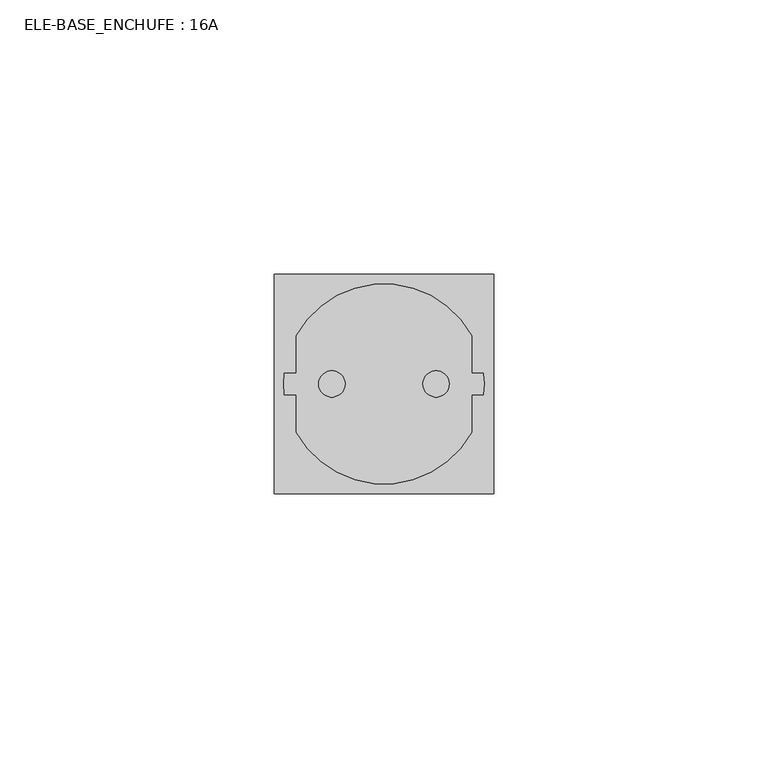
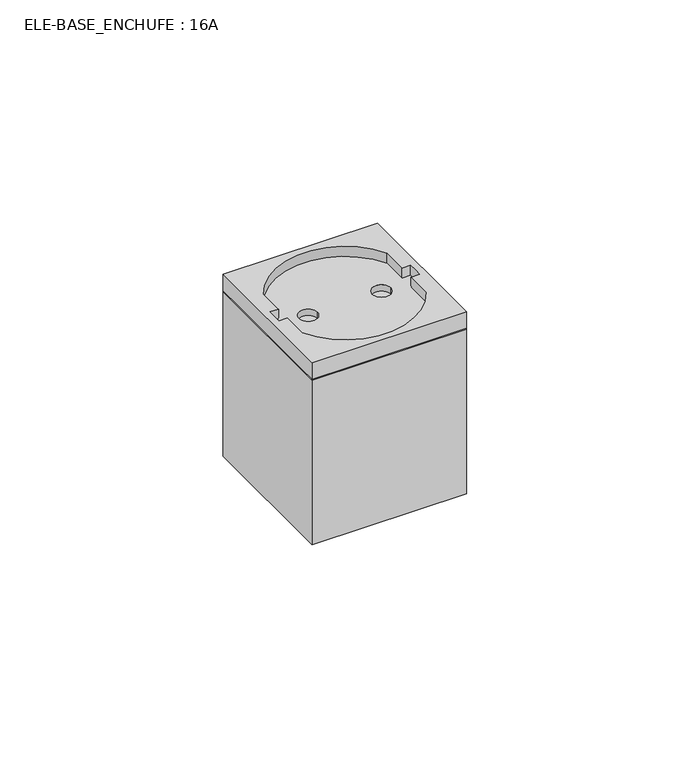
"""IFC4 building model written with IfcOpenShell, lengths in millimetres: proxy geometry, ELE-BASE_ENCHUFE : 16A."""

from ifc_helpers import new_model, si_unit, frame, origin, place, context, project, spatial, polyline, circle_curve, outline, extrude, source, transform, mapped, element, save
from ifc_brep_helpers import plane_surface, revolved_surface, advanced_brep


def ele_base_enchufe_16a_16eab72e(model_context):
    return source(origin(), model_context, "Body", "SolidModel", [
        extrude(outline(polyline([(20.0, 20.0), (20.0, -20.0), (-20.0, -20.0), (-20.0, 20.0), (20.0, 20.0)])), frame((0.0, 0.0, -45.0), z_axis=(0.0, 0.0, 1.0), x_axis=(1.0, 0.0, 0.0)), (0.0, 0.0, 1.0), 45.0),
        advanced_brep(
        [(20.0, 20.0, 4.7625), (-20.0, 20.0, 4.7625), (-20.0, -20.0, 4.7625), (20.0, -20.0, 4.7625), (-16.0, -8.7785249, 4.7625), (-16.0, -2.0, 4.7625), (-18.1400799, -2.0, 4.7625), (-18.1400799, 2.0, 4.7625), (-16.0, 2.0, 4.7625), (-16.0, 8.7785249, 4.7625), (16.0, 8.7785249, 4.7625), (16.0, 2.0, 4.7625), (18.1400799, 2.0, 4.7625), (18.1400799, -2.0, 4.7625), (16.0, -2.0, 4.7625), (16.0, -8.7785249, 4.7625), (20.0, 20.0, 0.0), (20.0, -20.0, 0.0), (-20.0, -20.0, 0.0), (-20.0, 20.0, 0.0), (-11.9, 0.0, 0.0), (-7.1, 0.0, 0.0), (7.1, 0.0, 0.0), (11.9, 0.0, 0.0), (-16.0, -2.0, 2.0), (-16.0, -8.7785249, 2.0), (16.0, -8.7785249, 2.0), (16.0, -2.0, 2.0), (18.1400799, -2.0, 2.0), (18.1400799, 2.0, 2.0), (16.0, 2.0, 2.0), (16.0, 8.7785249, 2.0), (-16.0, 8.7785249, 2.0), (-16.0, 2.0, 2.0), (-18.1400799, 2.0, 2.0), (-18.1400799, -2.0, 2.0), (-7.1, 0.0, 2.0), (-11.9, 0.0, 2.0), (11.9, 0.0, 2.0), (7.1, 0.0, 2.0)],
        [
            (0, 1),
            (1, 2),
            (2, 3),
            (3, 0),
            (4, 5),
            (5, 6),
            (6, 7, circle_curve(frame((0.0, 0.0, 4.7625), z_axis=(0.0, 0.0, -1.0), x_axis=(1.0, 0.0, 0.0)), 18.25)),
            (7, 8),
            (8, 9),
            (9, 10, circle_curve(frame((0.0, 0.0, 4.7625), z_axis=(0.0, 0.0, -1.0), x_axis=(1.0, 0.0, 0.0)), 18.25)),
            (10, 11),
            (11, 12),
            (12, 13, circle_curve(frame((0.0, 0.0, 4.7625), z_axis=(0.0, 0.0, -1.0), x_axis=(1.0, 0.0, 0.0)), 18.25)),
            (13, 14),
            (14, 15),
            (15, 4, circle_curve(frame((0.0, 0.0, 4.7625), z_axis=(0.0, 0.0, -1.0), x_axis=(1.0, 0.0, 0.0)), 18.25)),
            (16, 17),
            (17, 18),
            (18, 19),
            (19, 16),
            (20, 21, circle_curve(frame((-9.5, 0.0, 0.0), z_axis=(0.0, 0.0, 1.0), x_axis=(1.0, 0.0, 0.0)), 2.4)),
            (21, 20, circle_curve(frame((-9.5, 0.0, 0.0), z_axis=(0.0, 0.0, 1.0), x_axis=(1.0, 0.0, 0.0)), 2.4)),
            (22, 23, circle_curve(frame((9.5, 0.0, 0.0), z_axis=(0.0, 0.0, 1.0), x_axis=(1.0, 0.0, 0.0)), 2.4)),
            (23, 22, circle_curve(frame((9.5, 0.0, 0.0), z_axis=(0.0, 0.0, 1.0), x_axis=(1.0, 0.0, 0.0)), 2.4)),
            (0, 16),
            (19, 1),
            (18, 2),
            (17, 3),
            (24, 25),
            (25, 26, circle_curve(frame((0.0, 0.0, 2.0), z_axis=(0.0, 0.0, 1.0), x_axis=(1.0, 0.0, 0.0)), 18.25)),
            (26, 27),
            (27, 28),
            (28, 29, circle_curve(frame((0.0, 0.0, 2.0), z_axis=(0.0, 0.0, 1.0), x_axis=(1.0, 0.0, 0.0)), 18.25)),
            (29, 30),
            (30, 31),
            (31, 32, circle_curve(frame((0.0, 0.0, 2.0), z_axis=(0.0, 0.0, 1.0), x_axis=(1.0, 0.0, 0.0)), 18.25)),
            (32, 33),
            (33, 34),
            (34, 35, circle_curve(frame((0.0, 0.0, 2.0), z_axis=(0.0, 0.0, 1.0), x_axis=(1.0, 0.0, 0.0)), 18.25)),
            (35, 24),
            (36, 37, circle_curve(frame((-9.5, 0.0, 2.0), z_axis=(0.0, 0.0, -1.0), x_axis=(1.0, 0.0, 0.0)), 2.4)),
            (37, 36, circle_curve(frame((-9.5, 0.0, 2.0), z_axis=(0.0, 0.0, -1.0), x_axis=(1.0, 0.0, 0.0)), 2.4)),
            (38, 39, circle_curve(frame((9.5, 0.0, 2.0), z_axis=(0.0, 0.0, -1.0), x_axis=(1.0, 0.0, 0.0)), 2.4)),
            (39, 38, circle_curve(frame((9.5, 0.0, 2.0), z_axis=(0.0, 0.0, -1.0), x_axis=(1.0, 0.0, 0.0)), 2.4)),
            (24, 5),
            (4, 25),
            (15, 26),
            (14, 27),
            (13, 28),
            (12, 29),
            (11, 30),
            (10, 31),
            (9, 32),
            (8, 33),
            (7, 34),
            (6, 35),
            (20, 37),
            (36, 21),
            (22, 39),
            (38, 23),
        ],
        [
            plane_surface(frame((-40.0, 20.0, 4.7625), z_axis=(0.0, 0.0, 1.0), x_axis=(-1.0, 0.0, 0.0))),
            plane_surface(frame((-40.0, 20.0, 0.0), z_axis=(0.0, 0.0, -1.0), x_axis=(1.0, 0.0, 0.0))),
            plane_surface(frame((20.0, 20.0, 4.7625), z_axis=(0.0, 1.0, 0.0), x_axis=(0.0, 0.0, -1.0))),
            plane_surface(frame((-20.0, 20.0, 4.7625), z_axis=(-1.0, 0.0, 0.0), x_axis=(0.0, 0.0, -1.0))),
            plane_surface(frame((-20.0, -20.0, 4.7625), z_axis=(0.0, -1.0, 0.0), x_axis=(0.0, 0.0, -1.0))),
            plane_surface(frame((20.0, -20.0, 4.7625), z_axis=(1.0, 0.0, 0.0), x_axis=(0.0, 0.0, -1.0))),
            plane_surface(frame((-16.0, -8.7785249, 2.0), z_axis=(0.0, 0.0, 1.0), x_axis=(0.0, 1.0, 0.0))),
            plane_surface(frame((-16.0, -2.0, 4.8), z_axis=(1.0, 0.0, 0.0), x_axis=(0.0, 0.0, -1.0))),
            revolved_surface(polyline([(18.25, 0.0, 4.7625), (18.25, 0.0, 2.0)]), (0.0, 0.0, 2.0), (0.0, 0.0, 1.0)),
            plane_surface(frame((16.0, -8.7785249, 4.8), z_axis=(-1.0, 0.0, 0.0), x_axis=(0.0, 0.0, -1.0))),
            plane_surface(frame((16.0, -2.0, 4.8), z_axis=(0.0, 1.0, 0.0), x_axis=(0.0, 0.0, -1.0))),
            plane_surface(frame((18.1400799, 2.0, 4.8), z_axis=(0.0, -1.0, 0.0), x_axis=(0.0, 0.0, -1.0))),
            plane_surface(frame((16.0, 2.0, 4.8), z_axis=(-1.0, 0.0, 0.0), x_axis=(0.0, 0.0, -1.0))),
            plane_surface(frame((-16.0, 8.7785249, 4.8), z_axis=(1.0, 0.0, 0.0), x_axis=(0.0, 0.0, -1.0))),
            plane_surface(frame((-16.0, 2.0, 4.8), z_axis=(0.0, -1.0, 0.0), x_axis=(0.0, 0.0, -1.0))),
            plane_surface(frame((-18.1400799, -2.0, 4.8), z_axis=(0.0, 1.0, 0.0), x_axis=(0.0, 0.0, -1.0))),
            revolved_surface(polyline([(-7.1, 0.0, 2.0), (-7.1, 0.0, 0.0)]), (-9.5, 0.0, -18.0), (0.0, 0.0, 1.0)),
            revolved_surface(polyline([(11.9, 0.0, 2.0), (11.9, 0.0, 0.0)]), (9.5, 0.0, 0.0), (0.0, 0.0, 1.0)),
        ],
        [
            (0, [[1, 2, 3, 4], [5, 6, 7, 8, 9, 10, 11, 12, 13, 14, 15, 16]]),
            (1, [[17, 18, 19, 20], [21, 22], [23, 24]]),
            (2, [[-1, 25, -20, 26]]),
            (3, [[-2, -26, -19, 27]]),
            (4, [[-3, -27, -18, 28]]),
            (5, [[-4, -28, -17, -25]]),
            (6, [[29, 30, 31, 32, 33, 34, 35, 36, 37, 38, 39, 40], [41, 42], [43, 44]]),
            (7, [[-29, 45, -5, 46]]),
            (8, [[-30, -46, -16, 47]]),
            (9, [[-31, -47, -15, 48]]),
            (10, [[-32, -48, -14, 49]]),
            (8, [[-33, -49, -13, 50]]),
            (11, [[-34, -50, -12, 51]]),
            (12, [[-35, -51, -11, 52]]),
            (8, [[-36, -52, -10, 53]]),
            (13, [[-37, -53, -9, 54]]),
            (14, [[-38, -54, -8, 55]]),
            (8, [[-39, -55, -7, 56]]),
            (15, [[-40, -56, -6, -45]]),
            (16, [[57, -41, 58, -21]]),
            (16, [[-57, -22, -58, -42]]),
            (17, [[59, -43, 60, -23]]),
            (17, [[-59, -24, -60, -44]]),
        ],
    ),
    ])


if __name__ == "__main__":
    model = new_model("IFC4")
    model_context = context("Model", 3, world=origin())
    ifc_project = project(units=[si_unit("LENGTHUNIT", "METRE", prefix="MILLI")], contexts=[model_context])
    site = spatial("IfcSite", under=ifc_project)
    building = spatial("IfcBuilding", under=site)
    placement = place(None, origin())
    ele_base_enchufe_16a_shape = ele_base_enchufe_16a_16eab72e(model_context)
    element("IfcBuildingElementProxy", 1, Name="ELE-BASE_ENCHUFE : 16A", ObjectType="ELE-BASE_ENCHUFE : 16A", at=placement, inside=building, context=model_context, shape_type="MappedRepresentation", body=[
        mapped(ele_base_enchufe_16a_shape, transform((0.0, 0.0, 0.0), x_axis=(1.0, 0.0, 0.0), y_axis=(0.0, 1.0, 0.0), z_axis=(0.0, 0.0, 1.0))),
    ])
    save(model, "model.ifc")

# Revit data of these elements
# Project information
#   Subproyecto = "Información de proyecto"
#   Fecha de emisión de proyecto = "Fecha de emisión"
#   Estado de proyecto = "Estado de proyecto"
#   Nombre de cliente = "Propietario"
#   Dirección de proyecto = "Introduzca dirección aquí"
#   Nombre de proyecto = "Nombre de proyecto"
#   Número de proyecto = "0001"
# Type "ELE-BASE_ENCHUFE : 16A"
#   Etiqueta = ""
#   Voltaje toma corriente = 230 V
#   SimboloPosicionVertical [instance default] = 0.05 m
#   SimboloPosicionHorizontal [instance default] = 0.00 m
#   Potencia = 3680 W
#   Intensidad = 16 A
#   Carga = 3680 VA
#   Default Elevation = 0.20 m
#   Altura = 0.20 m
#   Simbolo25A = no
#   Simbolo16AEstanco = no
#   Simbolo16A = yes
#   Clasificación de carga = Toma de corriente
#   Assembly Code = ""
